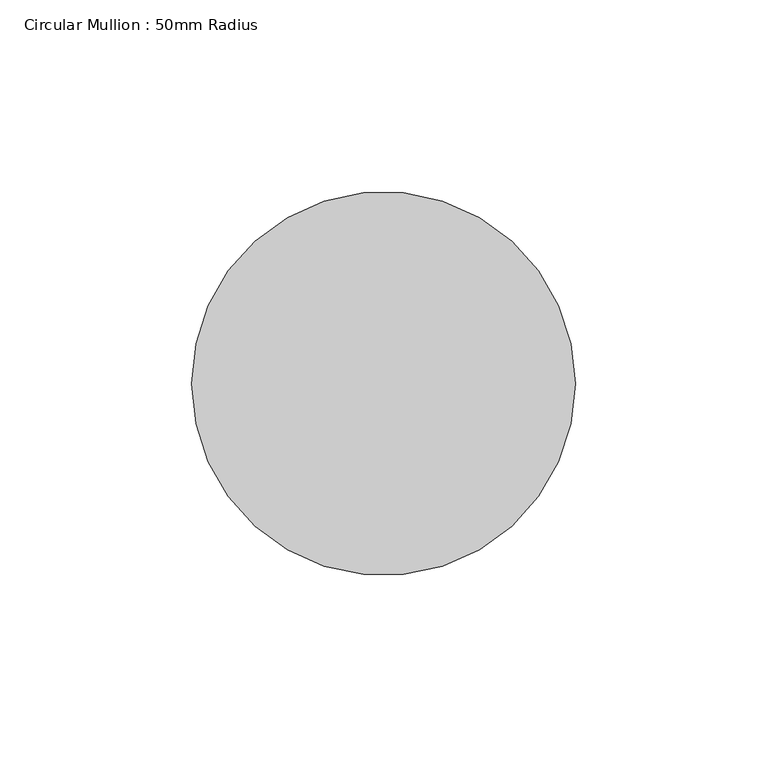
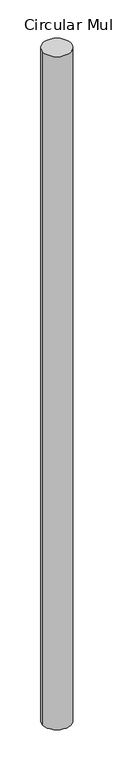
"""IFC4 building model written with IfcOpenShell, lengths in millimetres: member geometry, Circular Mullion : 50mm Radius."""

from ifc_helpers import new_model, si_unit, point, frame, frame_2d, origin, place, context, project, spatial, circle_curve, trimmed, segment, composite_curve, outline, extrude, source, transform, mapped, element, save


def circular_mullion_50mm_radius_ad7eff1a(model_context):
    return source(origin(), model_context, "Body", "SweptSolid", [
        extrude(outline(composite_curve([segment(trimmed(circle_curve(frame_2d((-50.0, 0.0)), 50.0), [point((0.0, 0.0))], [point((-100.0, 0.0))], False, "CARTESIAN"), True, "CONTINUOUS"), segment(trimmed(circle_curve(frame_2d((-50.0, 0.0)), 50.0), [point((-100.0, 0.0))], [point((0.0, 0.0))], False, "CARTESIAN"), True, "CONTINUOUS")], self_intersect=False)), frame((0.0, 0.0, -2557.0554245), z_axis=(0.0, 0.0, 1.0), x_axis=(1.0, 0.0, 0.0)), (0.0, 0.0, 1.0), 2557.0554245),
    ])


if __name__ == "__main__":
    model = new_model("IFC4")
    model_context = context("Model", 3, world=origin())
    ifc_project = project(units=[si_unit("LENGTHUNIT", "METRE", prefix="MILLI")], contexts=[model_context])
    site = spatial("IfcSite", under=ifc_project)
    building = spatial("IfcBuilding", under=site)
    placement = place(None, origin())
    circular_mullion_50mm_radius_shape = circular_mullion_50mm_radius_ad7eff1a(model_context)
    element("IfcMember", 1, ObjectType="Circular Mullion : 50mm Radius", at=placement, inside=building, context=model_context, shape_type="MappedRepresentation", body=[
        mapped(circular_mullion_50mm_radius_shape, transform((0.0, 0.0, 0.0), x_axis=(1.0, 0.0, 0.0), y_axis=(0.0, 1.0, 0.0), z_axis=(0.0, 0.0, 1.0))),
    ])
    save(model, "model.ifc")

# Revit data of these elements
# Type "Circular Mullion : 50mm Radius"
#   built-in parameter 1007350 = 0.164042 (stored number, unit not read)
# Element 1 (IfcMember, "Circular Mullion : 50mm Radius")
#   Materials on its faces: "Aluminium"
# Materials
#   "Aluminium": class "Metal", colour RGB 247 247 247, transparency 0, Description = "Aluminium 6061", Cost = 0
